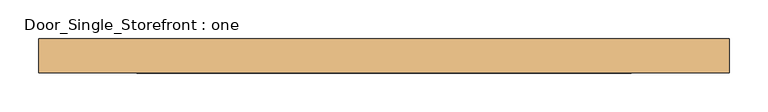
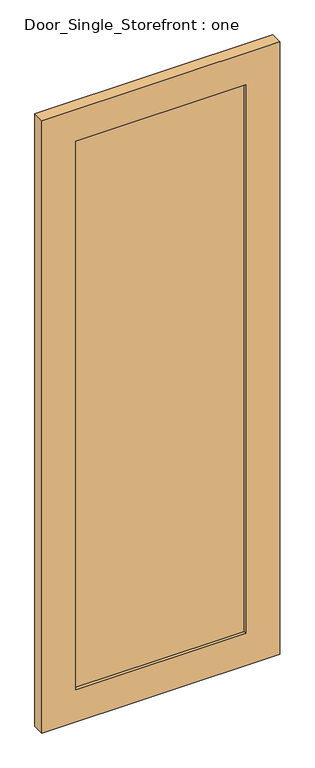
"""IFC4 building model written with IfcOpenShell, lengths in millimetres: door geometry, Door_Single_Storefront : one."""

from ifc_helpers import new_model, si_unit, frame, origin, place, context, project, spatial, polyline, outline, extrude, source, transform, mapped, element, save


def door_single_storefront_one_9c5224e2(model_context):
    return source(origin(), model_context, "Body", "SweptSolid", [
        extrude(outline(polyline([(319.88125, -6.35), (-319.88125, -6.35), (-319.88125, 12.7), (319.88125, 12.7), (319.88125, -6.35)])), frame((0.0, 0.0, 127.0), z_axis=(0.0, 0.0, 1.0), x_axis=(1.0, 0.0, 0.0)), (0.0, 0.0, 1.0), 2178.05),
        extrude(outline(polyline([(2432.05, -446.88125), (0.0, -446.88125), (0.0, 446.88125), (2432.05, 446.88125), (2432.05, -446.88125)]), holes=[polyline([(127.0, 319.88125), (127.0, -319.88125), (2305.05, -319.88125), (2305.05, 319.88125), (127.0, 319.88125)])]), frame((0.0, -19.05, 0.0), z_axis=(0.0, 1.0, 0.0), x_axis=(0.0, 0.0, 1.0)), (0.0, 0.0, 1.0), 44.45),
    ])


if __name__ == "__main__":
    model = new_model("IFC4")
    model_context = context("Model", 3, world=origin())
    ifc_project = project(units=[si_unit("LENGTHUNIT", "METRE", prefix="MILLI")], contexts=[model_context])
    site = spatial("IfcSite", under=ifc_project)
    building = spatial("IfcBuilding", under=site)
    placement = place(None, origin())
    door_single_storefront_one_shape = door_single_storefront_one_9c5224e2(model_context)
    element("IfcDoor", 1, ObjectType="Door_Single_Storefront : one", at=placement, inside=building, context=model_context, shape_type="MappedRepresentation", body=[
        mapped(door_single_storefront_one_shape, transform((0.0, 0.0, 0.0), x_axis=(1.0, 0.0, 0.0), y_axis=(0.0, 1.0, 0.0), z_axis=(0.0, 0.0, 1.0))),
    ])
    save(model, "model.ifc")

# Revit data of these elements
# Type "Door_Single_Storefront : one"
#   Type Mark = "27"
#   Analytic Construction = "<None>"
#   Stile_Width = 0' - 5"
#   Door_Thickness = 0' - 1 3/4"
#   Door_Offset = 0' - 1"
#   Glass_Material = SAFETY GLAZING
#   Frame_Material = INTERIOR GRADE ALUMINUM STOREFRONT W/ SAFETY GLAZING
#   Function = (empty or 0)
# Element 1 (IfcDoor, "Door_Single_Storefront : one")
#   Materials on its faces: "INTERIOR GRADE ALUMINUM STOREFRONT W/ SAFETY GLAZING", "SAFETY GLAZING"
# Materials
#   "SAFETY GLAZING": class "Glass", colour RGB 142 168 196, transparency 0.75, Description = "Soda Lime Glass", Cost = 0
#   "INTERIOR GRADE ALUMINUM STOREFRONT W/ SAFETY GLAZING": class "Metal", colour RGB 226 226 226, transparency 0, Description = "Aluminum 6061", Cost = 0
